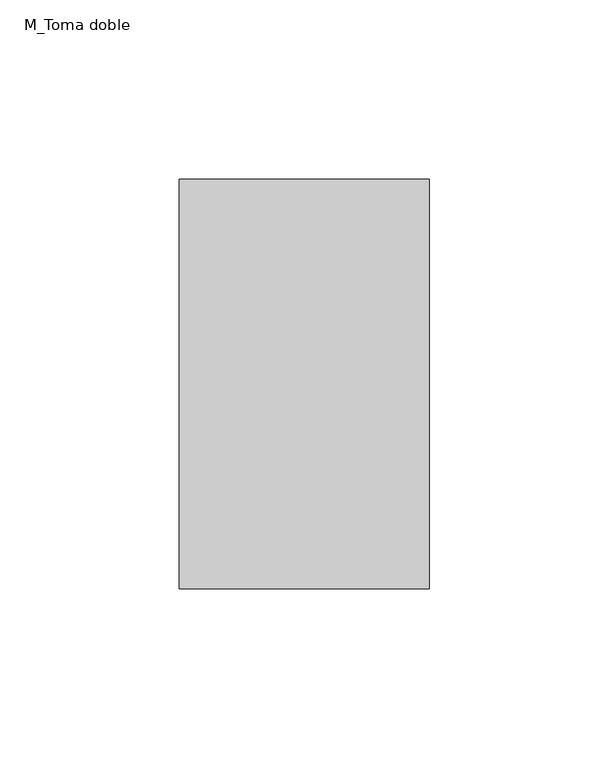
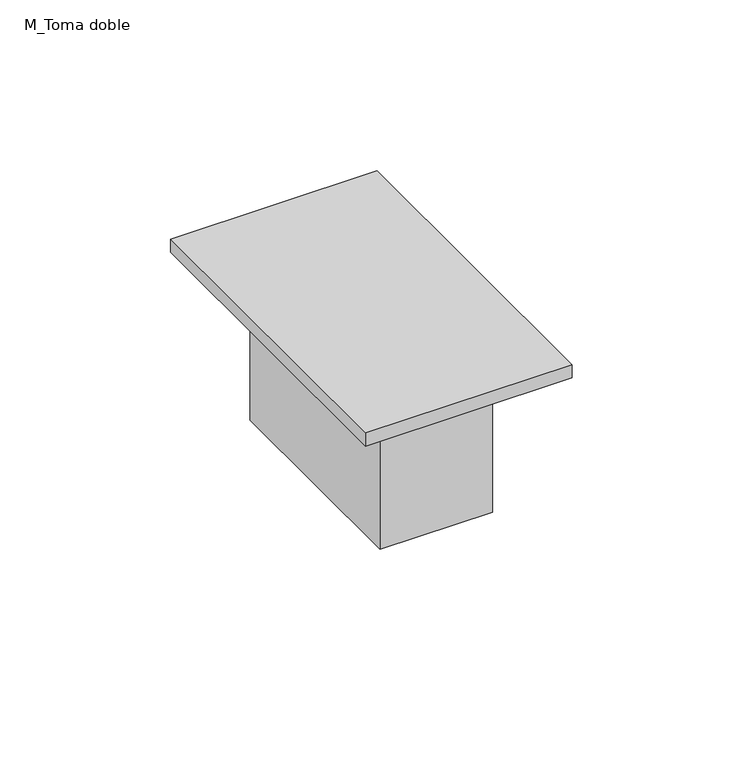
"""IFC4 building model written with IfcOpenShell, lengths in millimetres: proxy geometry, M_Toma doble : Estándar."""

from ifc_helpers import new_model, si_unit, frame, origin, origin_with_axes, place, context, project, spatial, polyline, outline, extrude, source, transform, mapped, element, save


def m_toma_doble_367a9a66(model_context):
    return source(origin(), model_context, "Body", "SweptSolid", [
        extrude(outline(polyline([(34.925, 57.15), (34.925, -57.15), (-34.925, -57.15), (-34.925, 57.15), (34.925, 57.15)])), origin_with_axes(), (0.0, 0.0, 1.0), 4.7625),
        extrude(outline(polyline([(19.05, 38.1), (19.05, -38.1), (-19.05, -38.1), (-19.05, 38.1), (19.05, 38.1)])), frame((0.0, 0.0, -53.975), z_axis=(0.0, 0.0, 1.0), x_axis=(1.0, 0.0, 0.0)), (0.0, 0.0, 1.0), 53.975),
    ])


if __name__ == "__main__":
    model = new_model("IFC4")
    model_context = context("Model", 3, world=origin())
    ifc_project = project(units=[si_unit("LENGTHUNIT", "METRE", prefix="MILLI")], contexts=[model_context])
    site = spatial("IfcSite", under=ifc_project)
    building = spatial("IfcBuilding", under=site)
    placement = place(None, origin())
    m_toma_doble_shape = m_toma_doble_367a9a66(model_context)
    element("IfcBuildingElementProxy", 1, Name="M_Toma doble : Estándar", ObjectType="M_Toma doble : Estándar", at=placement, inside=building, context=model_context, shape_type="MappedRepresentation", body=[
        mapped(m_toma_doble_shape, transform((0.0, 0.0, 0.0), x_axis=(1.0, 0.0, 0.0), y_axis=(0.0, 1.0, 0.0), z_axis=(0.0, 0.0, 1.0))),
    ])
    save(model, "model.ifc")

# Revit data of these elements
# Type "M_Toma doble : Estándar"
#   Texto de etiqueta = ""
#   Voltaje de interruptor = 120 V
#   Carga = 180 VA
#   Default Elevation = 0.46 m
#   Clasificación de carga = Toma de corriente
